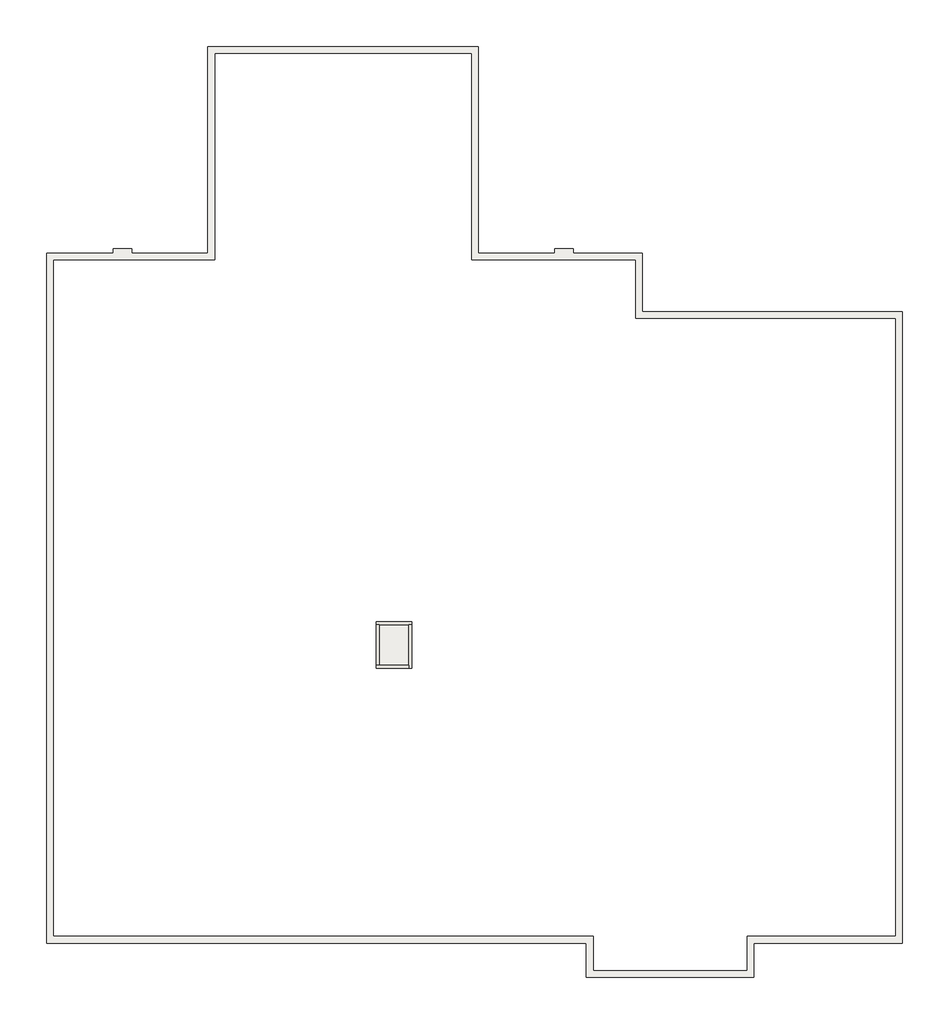
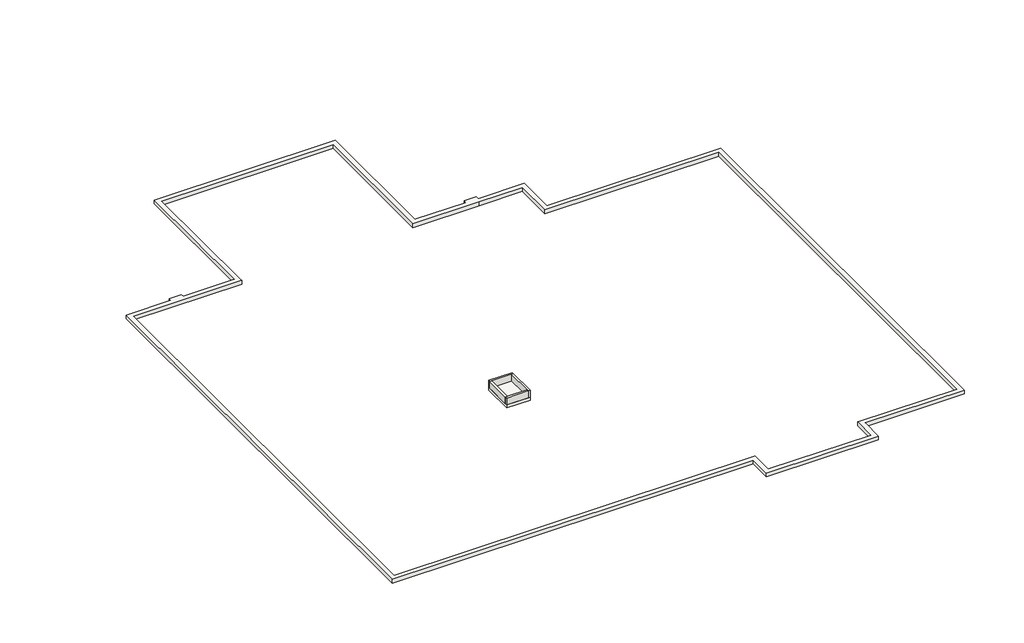
# One storey: 4 walls, 2 slabs.
"""IFC4 building model written with IfcOpenShell, lengths in millimetres."""

from ifc_helpers import new_model, si_unit, frame, origin, place, context, project, spatial, polyline, outline, extrude, faceted_brep, element, save

model = new_model("IFC4")

# Units and contexts
model_context = context("Model", 3, world=origin())
ifc_project = project(units=[si_unit("LENGTHUNIT", "METRE", prefix="MILLI")], contexts=[model_context])

# Site, building, storey
site = spatial("IfcSite", under=ifc_project)
building = spatial("IfcBuilding", under=site)
storey = spatial("IfcBuildingStorey", under=building, Name="02_FU_OKFU_-5,10__Aufzug", Elevation=-5100.0)

# Slabs
placement = place(None, origin())
element("IfcSlab", 1, ObjectType="5dki Aufzugsunterfahrt Bopla 40cm C40/50", at=placement, inside=storey, context=model_context, shape_type="SweptSolid", body=[
    extrude(outline(polyline([(30641.9991141, 10662.0130303), (30641.9991141, 6740.0014141), (27641.9992024, 6740.0014141), (27641.9992024, 10662.0130303), (30641.9991141, 10662.0130303)])), frame((0.0, 0.0, -5500.0), z_axis=(0.0, 0.0, 1.0), x_axis=(1.0, 0.0, 0.0)), (0.0, 0.0, 1.0), 400.0),
])
element("IfcSlab", 2, ObjectType="5dki Streifenfundament 50cm C100/115", at=placement, inside=storey, context=model_context, shape_type="SweptSolid", body=[
    extrude(outline(polyline([(13469.6232746, 59125.9283486), (36270.0003049, 59125.9283486), (36270.0003049, 41717.5032758), (42691.9991624, 41717.5032758), (42691.9991624, 42097.5032758), (44242.0014149, 42095.9282045), (44242.0014149, 41717.5032758), (50070.0000211, 41717.5032758), (50069.999894, 36785.573951), (71979.9986133, 36785.5734213), (71979.9986133, -16430.0005666), (59476.9100357, -16430.0005666), (59476.9100357, -19332.4966002), (45370.0202351, -19332.4966002), (45370.0202351, -16430.0005666), (-129.9986936, -16430.0005666), (-129.9986936, 41717.0011496), (5491.9984311, 41717.0011496), (5491.9984311, 42095.9291895), (7042.0004993, 42095.9291528), (7042.0004993, 41717.5032758), (13469.6232746, 41717.5032758), (13469.6232746, 59125.9283486)]), holes=[polyline([(35670.0003049, 58525.9283486), (14069.6232746, 58525.9283486), (14069.6232746, 41117.5032758), (470.0013064, 41117.5032758), (470.0013064, -15830.0005666), (45970.0202351, -15830.0005666), (45970.0202351, -18732.4966002), (58876.9100357, -18732.4966002), (58876.9100357, -15830.0005666), (71379.9986133, -15830.0005666), (71379.9986133, 36185.5734358), (49469.9998785, 36185.5739655), (49470.0000056, 41117.5032758), (44041.4717429, 41117.5032758), (35670.0003049, 41117.5032758), (35670.0003049, 58525.9283486)])]), frame((0.0, 0.0, -5100.0), z_axis=(0.0, 0.0, 1.0), x_axis=(1.0, 0.0, 0.0)), (0.0, 0.0, 1.0), 500.0),
])

# Walls
element("IfcWall", 3, ObjectType="5dki Aufzugsunterfahrt STB-Wand 25cm C40/50", at=placement, inside=storey, context=model_context, shape_type="Brep", body=[
    faceted_brep([(27641.9992024, 10412.0124709, -5100.0), (27891.9992024, 10412.0125176, -5100.0), (30385.8202349, 10412.0129836, -5100.0), (30635.8205887, 10412.0130303, -5100.0), (30635.8205887, 10412.0130303, -4200.0), (30385.8202349, 10412.0129836, -4200.0), (27891.9992024, 10412.0125176, -4200.0), (27641.9992024, 10412.0124709, -4200.0), (27641.9992024, 10662.0124709, -5100.0), (27641.9992024, 10662.0124709, -4200.0), (30635.3999388, 10662.0130303, -4200.0), (30635.3999388, 10662.0130303, -5100.0)], [[[0, 1, 2, 3, 4, 5, 6, 7]], [[8, 9, 10, 11]], [[3, 2, 1, 0, 8, 11]], [[7, 6, 5, 4, 10, 9]], [[4, 3, 11, 10]], [[0, 7, 9, 8]]]),
])
element("IfcWall", 4, ObjectType="5dki Aufzugsunterfahrt STB-Wand 25cm C40/50", at=placement, inside=storey, context=model_context, shape_type="Brep", body=[
    faceted_brep([(30385.8202349, 10412.0129836, -5100.0), (30391.5781103, 6990.0014141, -5100.0), (30391.9987602, 6740.0014141, -5100.0), (30391.9987602, 6740.0014141, -4200.0), (30391.5781103, 6990.0014141, -4200.0), (30385.8202349, 10412.0129836, -4200.0), (30635.8205887, 10412.0130303, -5100.0), (30635.8205887, 10412.0130303, -4200.0), (30641.9991141, 6740.0014141, -4200.0), (30641.9991141, 6740.0014141, -5100.0)], [[[0, 1, 2, 3, 4, 5]], [[6, 7, 8, 9]], [[2, 1, 0, 6, 9]], [[5, 4, 3, 8, 7]], [[0, 5, 7, 6]], [[3, 2, 9, 8]]]),
])
element("IfcWall", 5, ObjectType="5dki Aufzugsunterfahrt STB-Wand 25cm C40/50", at=placement, inside=storey, context=model_context, shape_type="Brep", body=[
    faceted_brep([(30391.5781103, 6990.0014141, -5100.0), (27891.9992024, 6990.0014141, -5100.0), (27641.9992024, 6990.0014141, -5100.0), (27641.9992024, 6990.0014141, -4200.0), (27891.9992024, 6990.0014141, -4200.0), (30391.5781103, 6990.0014141, -4200.0), (30391.9987602, 6740.0014141, -5100.0), (30391.9987602, 6740.0014141, -4200.0), (27641.9992024, 6740.0014141, -4200.0), (27641.9992024, 6740.0014141, -5100.0)], [[[0, 1, 2, 3, 4, 5]], [[6, 7, 8, 9]], [[2, 1, 0, 6, 9]], [[5, 4, 3, 8, 7]], [[0, 5, 7, 6]], [[3, 2, 9, 8]]]),
])
element("IfcWall", 6, ObjectType="5dki Aufzugsunterfahrt STB-Wand 25cm C40/50", at=placement, inside=storey, context=model_context, shape_type="SweptSolid", body=[
    extrude(outline(polyline([(27891.9992024, 10412.0125176), (27891.9992024, 6990.0014141), (27641.9992024, 6990.0014141), (27641.9992024, 10412.0124709), (27891.9992024, 10412.0125176)])), frame((0.0, 0.0, -5100.0), z_axis=(0.0, 0.0, 1.0), x_axis=(1.0, 0.0, 0.0)), (0.0, 0.0, 1.0), 900.0),
])

save(model, "model.ifc")

# Revit data of these elements
# Project information
#   StoreyModel = "<?xml version=\"1.0\" encoding=\"utf-16\"?>\n<StoreyModel xmlns:xsd=\"http://www.w3.org/2001/XMLSchema\" xmlns:xsi=\"http://www.w3.org/2001/XMLSchema-instance\" FormatVersion=\"2013.0.1.0\">\n  <GUID>d780c1b4-dd28-4844-915e-88a2c4b9528b</GUID>\n  <StoreyList />\n  <HelpLevelList />\n  <LastModificationDate>2014-08-27T10:30:40.9523468+02:00</LastModificationDate>\n  <LastModificationAutor>BiesingerMar</LastModificationAutor>\n  <SynchronizedStoreyModelFile />\n  <StandardConfiguration>\n    <Name>5D Standard</Name>\n    <Version>November 2012</Version>\n    <Description>5D-Standardkonfiguration</Description>\n    <LastModificationDate>2012-11-26T14:42:43.0850171+01:00</LastModificationDate>\n    <LastModificationAutor>5D-Administrator</LastModificationAutor>\n    <LevelStandard>\n      <LevelUsageList>\n        <LevelUsage>\n          <ID>0</ID>\n          <Function>Standard</Function>\n          <Name>STRD</Name>\n          <Abbreviation>STRD</Abbreviation>\n        </LevelUsage>\n        <LevelUsage>\n          <ID>1</ID>\n          <Function>Unterkante Rohdecke</Function>\n          <Name>UKRD</Name>\n          <Abbreviation>UKRD</Abbreviation>\n        </LevelUsage>\n        <LevelUsage>\n          <ID>2</ID>\n          <Function>Oberkante Rohdecke</Function>\n          <Name>OKRD</Name>\n          <Abbreviation>OKRD</Abbreviation>\n        </LevelUsage>\n        <LevelUsage>\n          <ID>3</ID>\n          <Function>Oberkante Fertigfußboden</Function>\n          <Name>OKFB</Name>\n          <Abbreviation>OKFB</Abbreviation>\n        </LevelUsage>\n        <LevelUsage>\n          <ID>4</ID>\n          <Function>Unterkante Abgehängter Decke</Function>\n          <Name>UKAD</Name>\n          <Abbreviation>UKAD</Abbreviation>\n        </LevelUsage>\n        <LevelUsage>\n          <ID>5</ID>\n          <Function>Statik</Function>\n          <Name>STAT</Name>\n          <Abbreviation>STAT</Abbreviation>\n        </LevelUsage>\n        <LevelUsage>\n          <ID>100</ID>\n          <Function>Hilfsebene</Function>\n          <Name>HELP</Name>\n          <Abbreviation>HELP</Abbreviation>\n        </LevelUsage>\n        <LevelUsage>\n          <ID>1000</ID>\n          <Function>Oberkante Fundament</Function>\n          <Name>OKFU</Name>\n          <Abbreviation>OKFU</Abbreviation>\n        </LevelUsage>\n        <LevelUsage>\n          <ID>1001</ID>\n          <Function>Unterkante Träger</Function>\n          <Name>UKTR</Name>\n          <Abbreviation>UKTR</Abbreviation>\n        </LevelUsage>\n        <LevelUsage>\n          <ID>1002</ID>\n          <Function>Lift</Function>\n          <Name>LIFT</Name>\n          <Abbreviation>LIFT</Abbreviation>\n        </LevelUsage>\n        <LevelUsage>\n          <ID>1003</ID>\n          <Function>Sockel</Function>\n          <Name>SOCK</Name>\n          <Abbreviation>SOCK</Abbreviation>\n        </LevelUsage>\n        <LevelUsage>\n          <ID>1004</ID>\n          <Function>Wandoberkante</Function>\n          <Name>OKWA</Name>\n          <Abbreviation>OKWA</Abbreviation>\n        </LevelUsage>\n        <LevelUsage>\n          <ID>1005</ID>\n          <Function>Dämmebene</Function>\n          <Name>DAEM</Name>\n          <Abbreviation>DAEM</Abbreviation>\n        </LevelUsage>\n        <LevelUsage>\n          <ID>1006</ID>\n          <Function>OK geneigtes Objekt</Function>\n          <Name>NEIG</Name>\n          <Abbreviation>NEIG</Abbreviation>\n        </LevelUsage>\n        <LevelUsage>\n          <ID>1007</ID>\n          <Function>Außenanlagen</Function>\n          <Name>AUSS</Name>\n          <Abbreviation>AUSS</Abbreviation>\n        </LevelUsage>\n        <LevelUsage>\n          <ID>1008</ID>\n          <Function>Boeschung Oberkante</Function>\n          <Name>BOOK</Name>\n          <Abbreviation>BOOK</Abbreviation>\n        </LevelUsage>\n        <LevelUsage>\n          <ID>1009</ID>\n          <Function>Boeschung Unterkante</Function>\n          <Name>BOUK</Name>\n          <Abbreviation>BOUK</Abbreviation>\n        </LevelUsage>\n        <LevelUsage>\n          <ID>1010</ID>\n          <Function>Treppe OK obere Ebene</Function>\n          <Name>TROK</Name>\n          <Abbreviation>TROK</Abbreviation>\n        </LevelUsage>\n        <LevelUsage>\n          <ID>1011</ID>\n          <Function>Treppe OK untere Ebene</Function>\n          <Name>TRUK</Name>\n          <Abbreviation>TRUK</Abbreviation>\n        </LevelUsage>\n        <LevelUsage>\n          <ID>1012</ID>\n          <Function>Treppe OK Podest 1</Function>\n          <Name>TRP1</Name>\n          <Abbreviation>TRP1</Abbreviation>\n        </LevelUsage>\n        <LevelUsage>\n          <ID>1013</ID>\n          <Function>Treppe OK Podest 2</Function>\n          <Name>TRP2</Name>\n          <Abbreviation>TRP2</Abbreviation>\n        </LevelUsage>\n        <LevelUsage>\n          <ID>1014</ID>\n          <Function>Unterkante Fundament</Function>\n          <Name>UKFU</Name>\n          <Abbreviation>UKFU</Abbreviation>\n        </LevelUsage>\n        <LevelUsage>\n          <ID>1015</ID>\n          <Function>Attika OK</Function>\n          <Name>ATOK</Name>\n          <Abbreviation>ATOK</Abbreviation>\n        </LevelUsage>\n        <LevelUsage>\n          <ID>1017</ID>\n          <Function>OK Vormauerung</Function>\n          <Name>OKVM</Name>\n          <Abbreviation>OKVM</Abbreviation>\n        </LevelUsage>\n        <LevelUsage>\n          <ID>1018</ID>\n          <Function>Lichtschacht Oberkante</Function>\n          <Name>LISO</Name>\n          <Abbreviation>LISO</Abbreviation>\n        </LevelUsage>\n        <LevelUsage>\n          <ID>1019</ID>\n          <Function>Unterkante Dämmung</Function>\n          <Name>DAEU</Name>\n          <Abbreviation>DAEU</Abbreviation>\n        </LevelUsage>\n      </LevelUsageList>\n      <DefaultLevelNameLogic>[Geschoss_FormatNummer]_[Geschoss_Verwendung_Kuerzel]_[Ebenen_Verwendung_Kuerzel]_[Ebenen_Projekthöhe]_[Ebenen_Kommentar]</DefaultLevelNameLogic>\n      <DefaultMainLevelUsage>3</DefaultMainLevelUsage>\n    </LevelStandard>\n    <StoreyStandard>\n      <DefaultStoreyNameLogic>[Geschoss_FormatNummer]_[Geschoss_Verwendung_Kuerzel]</DefaultStoreyNameLogic>\n      <StoreyUsageList>\n        <StoreyUsage>\n          <ID>0</ID>\n          <Function>Standard</Function>\n          <Name>Standard</Name>\n          <Abbreviation>ZZ</Abbreviation>\n        </StoreyUsage>\n        <StoreyUsage>\n          <ID>1</ID>\n          <Function>OberGeschoss</Function>\n          <Name>OberGeschoss</Name>\n          <Abbreviation>OG</Abbreviation>\n        </StoreyUsage>\n        <StoreyUsage>\n          <ID>2</ID>\n          <Function>UnterGeschoss</Function>\n          <Name>UnterGeschoss</Name>\n          <Abbreviation>UG</Abbreviation>\n        </StoreyUsage>\n        <StoreyUsage>\n          <ID>3</ID>\n          <Function>ErdGeschoss</Function>\n          <Name>ErdGeschoss</Name>\n          <Abbreviation>EG</Abbreviation>\n        </StoreyUsage>\n        <StoreyUsage>\n          <ID>4</ID>\n          <Function>DachGeschoss</Function>\n          <Name>DachGeschoss</Name>\n          <Abbreviation>DG</Abbreviation>\n        </StoreyUsage>\n        <StoreyUsage>\n          <ID>6</ID>\n          <Function>Keller</Function>\n          <Name>KellerGeschoss</Name>\n          <Abbreviation>KG</Abbreviation>\n        </StoreyUsage>\n        <StoreyUsage>\n          <ID>7</ID>\n          <Function>Tiefgarage</Function>\n          <Name>TiefgaragenGeschoss</Name>\n          <Abbreviation>TG</Abbreviation>\n        </StoreyUsage>\n        <StoreyUsage>\n          <ID>5</ID>\n          <Function>Technisches Geschoss</Function>\n          <Name>Technisches Geschoss</Name>\n          <Abbreviation>XG</Abbreviation>\n        </StoreyUsage>\n        <StoreyUsage>\n          <ID>1000</ID>\n          <Function>Treppenhaus</Function>\n          <Name>ZwischengGeschossTreppe</Name>\n          <Abbreviation>ZG</Abbreviation>\n        </StoreyUsage>\n        <StoreyUsage>\n          <ID>1001</ID>\n          <Function>Fundament</Function>\n          <Name>Fundament</Name>\n          <Abbreviation>FU</Abbreviation>\n        </StoreyUsage>\n        <StoreyUsage>\n          <ID>1002</ID>\n          <Function>Dachkonstruktion</Function>\n          <Name>Dachkonstruktion</Name>\n          <Abbreviation>DA</Abbreviation>\n        </StoreyUsage>\n        <StoreyUsage>\n          <ID>1004</ID>\n          <Function>Lift</Function>\n          <Name>Lift</Name>\n          <Abbreviation>LI</Abbreviation>\n        </StoreyUsage>\n      </StoreyUsageList>\n      <StoreyLocationList>\n        <StoreyLocation>\n          <ID>1</ID>\n          <Function>oberirdisch</Function>\n          <Name>oberirdisch</Name>\n          <Abbreviation />\n        </StoreyLocation>\n        <StoreyLocation>\n          <ID>2</ID>\n          <Function>unterirdisch</Function>\n          <Name>unterirdisch</Name>\n          <Abbreviation />\n        </StoreyLocation>\n      </StoreyLocationList>\n      <StoreyHeight>9.84251968503937</StoreyHeight>\n      <StoreyNumberOnOvergroundFormat>\n        <Digits>2</Digits>\n        <Prefix />\n        <Suffix />\n      </StoreyNumberOnOvergroundFormat>\n      <StoreyNumberOnUndergroundFormat>\n        <Digits>2</Digits>\n        <Prefix />\n        <Suffix />\n      </StoreyNumberOnUndergroundFormat>\n      <EntresolNumberFormat>\n        <Digits>2</Digits>\n        <Prefix />\n        <Suffix />\n      </EntresolNumberFormat>\n    </StoreyStandard>\n  </StandardConfiguration>\n  <RevisionNumber>35</RevisionNumber>\n  <WriteLock>false</WriteLock>\n</StoreyModel>"
#   BrowserStrukturXMLData = "<Browserstruktur>\n  <xs:schema id=\"Browserstruktur\" xmlns=\"\" xmlns:xs=\"http://www.w3.org/2001/XMLSchema\" xmlns:msdata=\"urn:schemas-microsoft-com:xml-msdata\">\n    <xs:element name=\"Browserstruktur\" msdata:IsDataSet=\"true\" msdata:MainDataTable=\"ViewTemplates\" msdata:UseCurrentLocale=\"true\">\n      <xs:complexType>\n        <xs:choice minOccurs=\"0\" maxOccurs=\"unbounded\">\n          <xs:element name=\"ViewTemplates\">\n            <xs:complexType>\n              <xs:sequence>\n                <xs:element name=\"Erstellen\" type=\"xs:boolean\" minOccurs=\"0\" />\n                <xs:element name=\"Ansichtsvorlage\" type=\"xs:string\" />\n                <xs:element name=\"_x0031__Fachbereich\" type=\"xs:string\" minOccurs=\"0\" />\n                <xs:element name=\"_x0032__Ansichtstyp\" type=\"xs:string\" minOccurs=\"0\" />\n                <xs:element name=\"_x0033__Ansichtsgruppe\" type=\"xs:string\" minOccurs=\"0\" />\n                <xs:element name=\"Typ\" type=\"xs:string\" minOccurs=\"0\" />\n                <xs:element name=\"Klasse\" type=\"xs:string\" minOccurs=\"0\" />\n                <xs:element name=\"Bedingung\" type=\"xs:string\" minOccurs=\"0\" />\n                <xs:element name=\"Ebenenbezug\" type=\"xs:int\" minOccurs=\"0\" />\n                <xs:element name=\"Ansichtsrichtung\" type=\"xs:string\" minOccurs=\"0\" />\n                <xs:element name=\"Ansichtsname\" type=\"xs:string\" minOccurs=\"0\" />\n              </xs:sequence>\n            </xs:complexType>\n          </xs:element>\n        </xs:choice>\n      </xs:complexType>\n      <xs:unique name=\"Constraint1\" msdata:PrimaryKey=\"true\">\n        <xs:selector xpath=\".//ViewTemplates\" />\n        <xs:field xpath=\"Ansichtsvorlage\" />\n      </xs:unique>\n    </xs:element>\n  </xs:schema>\n  <ViewTemplates>\n    <Erstellen>false</Erstellen>\n    <Ansichtsvorlage>010</Ansichtsvorlage>\n    <_x0031__Fachbereich>00_INTERN</_x0031__Fachbereich>\n    <_x0032__Ansichtstyp>010_CAD_UNTERLAGE</_x0032__Ansichtstyp>\n    <_x0033__Ansichtsgruppe>010_UNTERLAGE_CAD_GESAMT</_x0033__Ansichtsgruppe>\n    <Typ>FloorPlan</Typ>\n    <Klasse>ViewPlan</Klasse>\n    <Bedingung>einmalig</Bedingung>\n    <Ansichtsrichtung>&lt;Ignorieren&gt;</Ansichtsrichtung>\n    <Ansichtsname>[Geschoss_Name]_[Ansichtsgruppe_Name]_[Ebenen_Kommentar]</Ansichtsname>\n  </ViewTemplates>\n  <ViewTemplates>\n    <Erstellen>false</Erstellen>\n    <Ansichtsvorlage>011</Ansichtsvorlage>\n    <_x0031__Fachbereich>00_INTERN</_x0031__Fachbereich>\n    <_x0032__Ansichtstyp>010_CAD_UNTERLAGE</_x0032__Ansichtstyp>\n    <_x0033__Ansichtsgruppe>011_LAGEPLAN</_x0033__Ansichtsgruppe>\n    <Typ>FloorPlan</Typ>\n    <Klasse>ViewPlan</Klasse>\n    <Bedingung>einmalig</Bedingung>\n    <Ansichtsrichtung>&lt;Ignorieren&gt;</Ansichtsrichtung>\n    <Ansichtsname>[Geschoss_Name]_[Ansichtsgruppe_Name]_[Ebenen_Kommentar]</Ansichtsname>\n  </ViewTemplates>\n  <ViewTemplates>\n    <Erstellen>false</Erstellen>\n    <Ansichtsvorlage>025</Ansichtsvorlage>\n    <_x0031__Fachbereich>00_INTERN</_x0031__Fachbereich>\n    <_x0032__Ansichtstyp>010_CAD_UNTERLAGE</_x0032__Ansichtstyp>\n    <_x0033__Ansichtsgruppe>025_ACHSEN</_x0033__Ansichtsgruppe>\n    <Typ>FloorPlan</Typ>\n    <Klasse>ViewPlan</Klasse>\n    <Bedingung>einmalig</Bedingung>\n    <Ansichtsrichtung>&lt;Ignorieren&gt;</Ansichtsrichtung>\n    <Ansichtsname>[Geschoss_Name]_[Ansichtsgruppe_Name]_[Ebenen_Kommentar]</Ansichtsname>\n  </ViewTemplates>\n  <ViewTemplates>\n    <Erstellen>false</Erstellen>\n    <Ansichtsvorlage>030</Ansichtsvorlage>\n    <_x0031__Fachbereich>00_INTERN</_x0031__Fachbereich>\n    <_x0032__Ansichtstyp>010_CAD_UNTERLAGE</_x0032__Ansichtstyp>\n    <_x0033__Ansichtsgruppe>030_ENTWURF_ARCHITEKT</_x0033__Ansichtsgruppe>\n    <Typ>FloorPlan</Typ>\n    <Klasse>ViewPlan</Klasse>\n    <Bedingung>einmalig</Bedingung>\n    <Ebenenbezug>100</Ebenenbezug>\n    <Ansichtsrichtung>&lt;Ignorieren&gt;</Ansichtsrichtung>\n    <Ansichtsname>[Geschoss_Name]_[Ansichtsgruppe_Name]_[Ebenen_Kommentar]</Ansichtsname>\n  </ViewTemplates>\n  <ViewTemplates>\n    <Erstellen>false</Erstellen>\n    <Ansichtsvorlage>060</Ansichtsvorlage>\n    <_x0031__Fachbereich>00_INTERN</_x0031__Fachbereich>\n    <_x0032__Ansichtstyp>060_BILD_UNTERLAGE</_x0032__Ansichtstyp>\n    <_x0033__Ansichtsgruppe>060_UNTERLAGE_BITMAP</_x0033__Ansichtsgruppe>\n    <Typ>FloorPlan</Typ>\n    <Klasse>ViewPlan</Klasse>\n    <Bedingung>einmalig</Bedingung>\n    <Ansichtsrichtung>&lt;Ignorieren&gt;</Ansichtsrichtung>\n    <Ansichtsname>[Geschoss_Name]_[Ansichtsgruppe_Name]_[Ebenen_Kommentar]</Ansichtsname>\n  </ViewTemplates>\n  <ViewTemplates>\n    <Erstellen>false</Erstellen>\n    <Ansichtsvorlage>070</Ansichtsvorlage>\n    <_x0031__Fachbereich>00_INTERN</_x0031__Fachbereich>\n    <_x0032__Ansichtstyp>070_CAD_UEBERLAGE</_x0032__Ansichtstyp>\n    <_x0033__Ansichtsgruppe>070_UEBERLAGE_CAD</_x0033__Ansichtsgruppe>\n    <Typ>FloorPlan</Typ>\n    <Klasse>ViewPlan</Klasse>\n    <Bedingung>einmalig</Bedingung>\n    <Ansichtsrichtung>&lt;Ignorieren&gt;</Ansichtsrichtung>\n    <Ansichtsname>[Geschoss_Name]_[Ansichtsgruppe_Name]_[Ebenen_Kommentar]</Ansichtsname>\n  </ViewTemplates>\n  <ViewTemplates>\n    <Erstellen>false</Erstellen>\n    <Ansichtsvorlage>080</Ansichtsvorlage>\n    <_x0031__Fachbereich>00_INTERN</_x0031__Fachbereich>\n    <_x0032__Ansichtstyp>080_BILD_UEBERLAGE</_x0032__Ansichtstyp>\n    <_x0033__Ansichtsgruppe>080_UEBERLAGE_BITMAP</_x0033__Ansichtsgruppe>\n    <Typ>FloorPlan</Typ>\n    <Klasse>ViewPlan</Klasse>\n    <Bedingung>einmalig</Bedingung>\n    <Ansichtsrichtung>&lt;Ignorieren&gt;</Ansichtsrichtung>\n    <Ansichtsname>[Geschoss_Name]_[Ansichtsgruppe_Name]_[Ebenen_Kommentar]</Ansichtsname>\n  </ViewTemplates>\n  <ViewTemplates>\n    <Erstellen>false</Erstellen>\n    <Ansichtsvorlage>K_5_CC</Ansichtsvorlage>\n    <_x0031__Fachbereich>K_KONSTRUKTION</_x0031__Fachbereich>\n    <_x0032__Ansichtstyp>5_INGENIEUR / ROHBAU</_x0032__Ansichtstyp>\n    <_x0033__Ansichtsgruppe>5_CC_WÄNDE/STÜTZEN</_x0033__Ansichtsgruppe>\n    <Typ>FloorPlan</Typ>\n    <Klasse>ViewPlan</Klasse>\n    <Bedingung>Für jedes Geschoß</Bedingung>\n    <Ebenenbezug>-2</Ebenenbezug>\n    <Ansichtsrichtung>&lt;Ignorieren&gt;</Ansichtsrichtung>\n    <Ansichtsname>[Geschoss_Name]_[Ansichtsgruppe_Name]_[Ebenen_Kommentar]</Ansichtsname>\n  </ViewTemplates>\n  <ViewTemplates>\n    <Erstellen>false</Erstellen>\n    <Ansichtsvorlage>K_5_AA</Ansichtsvorlage>\n    <_x0031__Fachbereich>K_KONSTRUKTION</_x0031__Fachbereich>\n    <_x0032__Ansichtstyp>5_INGENIEUR / ROHBAU</_x0032__Ansichtstyp>\n    <_x0033__Ansichtsgruppe>5_AA_FUNDAMENTE</_x0033__Ansichtsgruppe>\n    <Typ>FloorPlan</Typ>\n    <Klasse>ViewPlan</Klasse>\n    <Bedingung>Für jedes Geschoß</Bedingung>\n    <Ebenenbezug>1000</Ebenenbezug>\n    <Ansichtsrichtung>&lt;Ignorieren&gt;</Ansichtsrichtung>\n    <Ansichtsname>[Geschoss_Name]_[Ansichtsgruppe_Name]_[Ebenen_Kommentar]</Ansichtsname>\n  </ViewTemplates>\n  <ViewTemplates>\n    <Erstellen>false</Erstellen>\n    <Ansichtsvorlage>K_5_BB</Ansichtsvorlage>\n    <_x0031__Fachbereich>K_KONSTRUKTION</_x0031__Fachbereich>\n    <_x0032__Ansichtstyp>5_INGENIEUR / ROHBAU</_x0032__Ansichtstyp>\n    <_x0033__Ansichtsgruppe>5_BB_BODENPLATTE</_x0033__Ansichtsgruppe>\n    <Typ>FloorPlan</Typ>\n    <Klasse>ViewPlan</Klasse>\n    <Bedingung>Für jedes Geschoß</Bedingung>\n    <Ebenenbezug>2</Ebenenbezug>\n    <Ansichtsrichtung>&lt;Ignorieren&gt;</Ansichtsrichtung>\n    <Ansichtsname>[Geschoss_Name]_[Ansichtsgruppe_Name]_[Ebenen_Kommentar]</Ansichtsname>\n  </ViewTemplates>\n  <ViewTemplates>\n    <Erstellen>false</Erstellen>\n    <Ansichtsvorlage>K_5_EE</Ansichtsvorlage>\n    <_x0031__Fachbereich>K_KONSTRUKTION</_x0031__Fachbereich>\n    <_x0032__Ansichtstyp>5_INGENIEUR / ROHBAU</_x0032__Ansichtstyp>\n    <_x0033__Ansichtsgruppe>5_EE_GESCHOSSDECKEN</_x0033__Ansichtsgruppe>\n    <Typ>FloorPlan</Typ>\n    <Klasse>ViewPlan</Klasse>\n    <Bedingung>Für jedes Geschoß</Bedingung>\n    <Ebenenbezug>2</Ebenenbezug>\n    <Ansichtsrichtung>&lt;Ignorieren&gt;</Ansichtsrichtung>\n    <Ansichtsname>[Geschoss_Name]_[Ansichtsgruppe_Name]_[Ebenen_Kommentar]</Ansichtsname>\n  </ViewTemplates>\n  <ViewTemplates>\n    <Erstellen>false</Erstellen>\n    <Ansichtsvorlage>K_6b_AA</Ansichtsvorlage>\n    <_x0031__Fachbereich>K_KONSTRUKTION</_x0031__Fachbereich>\n    <_x0032__Ansichtstyp>6b_FASSADE</_x0032__Ansichtstyp>\n    <_x0033__Ansichtsgruppe>6b_AA_FENSTER_UND_GLASFASSADE</_x0033__Ansichtsgruppe>\n    <Typ>FloorPlan</Typ>\n    <Klasse>ViewPlan</Klasse>\n    <Bedingung>Für jedes Geschoß</Bedingung>\n    <Ebenenbezug>-2</Ebenenbezug>\n    <Ansichtsrichtung>&lt;Ignorieren&gt;</Ansichtsrichtung>\n    <Ansichtsname>[Geschoss_Name]_[Ansichtsgruppe_Name]_[Ebenen_Kommentar]</Ansichtsname>\n  </ViewTemplates>\n  <ViewTemplates>\n    <Erstellen>false</Erstellen>\n    <Ansichtsvorlage>K_6b_DD</Ansichtsvorlage>\n    <_x0031__Fachbereich>K_KONSTRUKTION</_x0031__Fachbereich>\n    <_x0032__Ansichtstyp>6b_FASSADE</_x0032__Ansichtstyp>\n    <_x0033__Ansichtsgruppe>6b_DD_AUßENPUTZ_WDVS</_x0033__Ansichtsgruppe>\n    <Typ>FloorPlan</Typ>\n    <Klasse>ViewPlan</Klasse>\n    <Bedingung>Für jedes Geschoß</Bedingung>\n    <Ebenenbezug>-2</Ebenenbezug>\n    <Ansichtsrichtung>&lt;Ignorieren&gt;</Ansichtsrichtung>\n    <Ansichtsname>[Geschoss_Name]_[Ansichtsgruppe_Name]_[Ebenen_Kommentar]</Ansichtsname>\n  </ViewTemplates>\n  <ViewTemplates>\n    <Erstellen>false</Erstellen>\n    <Ansichtsvorlage>K_5_S1_AA</Ansichtsvorlage>\n    <_x0031__Fachbereich>K_KONSTRUKTION</_x0031__Fachbereich>\n    <_x0032__Ansichtstyp>5_S1_STATIK</_x0032__Ansichtstyp>\n    <_x0033__Ansichtsgruppe>5_S1_AA_GRUNDRISSE</_x0033__Ansichtsgruppe>\n    <Typ>FloorPlan</Typ>\n    <Klasse>ViewPlan</Klasse>\n    <Bedingung>Für jedes Geschoß</Bedingung>\n    <Ebenenbezug>-2</Ebenenbezug>\n    <Ansichtsrichtung>&lt;Ignorieren&gt;</Ansichtsrichtung>\n    <Ansichtsname>[Geschoss_Name]_[Ansichtsgruppe_Name]_[Ebenen_Kommentar]</Ansichtsname>\n  </ViewTemplates>\n  <ViewTemplates>\n    <Erstellen>false</Erstellen>\n    <Ansichtsvorlage>K_5_S2_AA</Ansichtsvorlage>\n    <_x0031__Fachbereich>K_KONSTRUKTION</_x0031__Fachbereich>\n    <_x0032__Ansichtstyp>5_S2_BEWEHRUNG</_x0032__Ansichtstyp>\n    <_x0033__Ansichtsgruppe>5_S2_AA_GRUNDRISSE</_x0033__Ansichtsgruppe>\n    <Typ>FloorPlan</Typ>\n    <Klasse>ViewPlan</Klasse>\n    <Bedingung>Für jedes Geschoß</Bedingung>\n    <Ebenenbezug>-2</Ebenenbezug>\n    <Ansichtsrichtung>&lt;Ignorieren&gt;</Ansichtsrichtung>\n    <Ansichtsname>[Geschoss_Name]_[Ansichtsgruppe_Name]_[Ebenen_Kommentar]</Ansichtsname>\n  </ViewTemplates>\n  <ViewTemplates>\n    <Erstellen>false</Erstellen>\n    <Ansichtsvorlage>K_5_DD</Ansichtsvorlage>\n    <_x0031__Fachbereich>K_KONSTRUKTION</_x0031__Fachbereich>\n    <_x0032__Ansichtstyp>5_INGENIEUR / ROHBAU</_x0032__Ansichtstyp>\n    <_x0033__Ansichtsgruppe>5_DD_TRÄGER</_x0033__Ansichtsgruppe>\n    <Typ>FloorPlan</Typ>\n    <Klasse>ViewPlan</Klasse>\n    <Bedingung>Für jedes Geschoß</Bedingung>\n    <Ebenenbezug>1</Ebenenbezug>\n    <Ansichtsrichtung>&lt;Ignorieren&gt;</Ansichtsrichtung>\n    <Ansichtsname>[Geschoss_Name]_[Ansichtsgruppe_Name]_[Ebenen_Kommentar]</Ansichtsname>\n  </ViewTemplates>\n  <ViewTemplates>\n    <Erstellen>false</Erstellen>\n    <Ansichtsvorlage>K_5_S1_BB</Ansichtsvorlage>\n    <_x0031__Fachbereich>K_KONSTRUKTION</_x0031__Fachbereich>\n    <_x0032__Ansichtstyp>5_S1_STATIK</_x0032__Ansichtstyp>\n    <_x0033__Ansichtsgruppe>5_S1_BB_DECKENSPIEGEL</_x0033__Ansichtsgruppe>\n    <Typ>FloorPlan</Typ>\n    <Klasse>ViewPlan</Klasse>\n    <Bedingung>Für jedes Geschoß</Bedingung>\n    <Ebenenbezug>2</Ebenenbezug>\n    <Ansichtsrichtung>&lt;Ignorieren&gt;</Ansichtsrichtung>\n    <Ansichtsname>[Geschoss_Name]_[Ansichtsgruppe_Name]_[Ebenen_Kommentar]</Ansichtsname>\n  </ViewTemplates>\n  <ViewTemplates>\n    <Erstellen>false</Erstellen>\n    <Ansichtsvor
#     lage>K_5_S2_BB</Ansichtsvorlage>\n    <_x0031__Fachbereich>K_KONSTRUKTION</_x0031__Fachbereich>\n    <_x0032__Ansichtstyp>5_S2_BEWEHRUNG</_x0032__Ansichtstyp>\n    <_x0033__Ansichtsgruppe>5_S2_BB_DECKENSPIEGEL</_x0033__Ansichtsgruppe>\n    <Typ>FloorPlan</Typ>\n    <Klasse>ViewPlan</Klasse>\n    <Bedingung>Für jedes Geschoß</Bedingung>\n    <Ebenenbezug>2</Ebenenbezug>\n    <Ansichtsrichtung>&lt;Ignorieren&gt;</Ansichtsrichtung>\n    <Ansichtsname>[Geschoss_Name]_[Ansichtsgruppe_Name]_[Ebenen_Kommentar]</Ansichtsname>\n  </ViewTemplates>\n  <ViewTemplates>\n    <Erstellen>false</Erstellen>\n    <Ansichtsvorlage>K_6b_BB</Ansichtsvorlage>\n    <_x0031__Fachbereich>K_KONSTRUKTION</_x0031__Fachbereich>\n    <_x0032__Ansichtstyp>6b_FASSADE</_x0032__Ansichtstyp>\n    <_x0033__Ansichtsgruppe>6b_BB_FASSADENBEKLEIDUNG</_x0033__Ansichtsgruppe>\n    <Typ>FloorPlan</Typ>\n    <Klasse>ViewPlan</Klasse>\n    <Bedingung>Für jedes Geschoß</Bedingung>\n    <Ebenenbezug>2</Ebenenbezug>\n    <Ansichtsrichtung>&lt;Ignorieren&gt;</Ansichtsrichtung>\n    <Ansichtsname>[Geschoss_Name]_[Ansichtsgruppe_Name]_[Ebenen_Kommentar]</Ansichtsname>\n  </ViewTemplates>\n  <ViewTemplates>\n    <Erstellen>false</Erstellen>\n    <Ansichtsvorlage>K_6b_CC</Ansichtsvorlage>\n    <_x0031__Fachbereich>K_KONSTRUKTION</_x0031__Fachbereich>\n    <_x0032__Ansichtstyp>6b_FASSADE</_x0032__Ansichtstyp>\n    <_x0033__Ansichtsgruppe>6b_CC_SONNENSCHUTZ_BLENDSCHUTZ</_x0033__Ansichtsgruppe>\n    <Typ>FloorPlan</Typ>\n    <Klasse>ViewPlan</Klasse>\n    <Bedingung>Für jedes Geschoß</Bedingung>\n    <Ebenenbezug>2</Ebenenbezug>\n    <Ansichtsrichtung>&lt;Ignorieren&gt;</Ansichtsrichtung>\n    <Ansichtsname>[Geschoss_Name]_[Ansichtsgruppe_Name]_[Ebenen_Kommentar]</Ansichtsname>\n  </ViewTemplates>\n  <ViewTemplates>\n    <Erstellen>false</Erstellen>\n    <Ansichtsvorlage>K_6c_AA</Ansichtsvorlage>\n    <_x0031__Fachbereich>K_KONSTRUKTION</_x0031__Fachbereich>\n    <_x0032__Ansichtstyp>6c_AUSBAU</_x0032__Ansichtstyp>\n    <_x0033__Ansichtsgruppe>6c_AA_WÄNDE_ALLGEMEIN</_x0033__Ansichtsgruppe>\n    <Typ>FloorPlan</Typ>\n    <Klasse>ViewPlan</Klasse>\n    <Bedingung>Für jedes Geschoß</Bedingung>\n    <Ebenenbezug>-2</Ebenenbezug>\n    <Ansichtsrichtung>&lt;Ignorieren&gt;</Ansichtsrichtung>\n    <Ansichtsname>[Geschoss_Name]_[Ansichtsgruppe_Name]_[Ebenen_Kommentar]</Ansichtsname>\n  </ViewTemplates>\n  <ViewTemplates>\n    <Erstellen>false</Erstellen>\n    <Ansichtsvorlage>K_6c_AC</Ansichtsvorlage>\n    <_x0031__Fachbereich>K_KONSTRUKTION</_x0031__Fachbereich>\n    <_x0032__Ansichtstyp>6c_AUSBAU</_x0032__Ansichtstyp>\n    <_x0033__Ansichtsgruppe>6c_AC_SYSTEMTRENNWÄNDE</_x0033__Ansichtsgruppe>\n    <Typ>FloorPlan</Typ>\n    <Klasse>ViewPlan</Klasse>\n    <Bedingung>Für jedes Geschoß</Bedingung>\n    <Ebenenbezug>3</Ebenenbezug>\n    <Ansichtsrichtung>&lt;Ignorieren&gt;</Ansichtsrichtung>\n    <Ansichtsname>[Geschoss_Name]_[Ansichtsgruppe_Name]_[Ebenen_Kommentar]</Ansichtsname>\n  </ViewTemplates>\n  <ViewTemplates>\n    <Erstellen>false</Erstellen>\n    <Ansichtsvorlage>K_6c_BX</Ansichtsvorlage>\n    <_x0031__Fachbereich>K_KONSTRUKTION</_x0031__Fachbereich>\n    <_x0032__Ansichtstyp>6c_AUSBAU</_x0032__Ansichtstyp>\n    <_x0033__Ansichtsgruppe>6c_BX_RÄUME (RAUMBEZEICHNUNGEN)</_x0033__Ansichtsgruppe>\n    <Typ>FloorPlan</Typ>\n    <Klasse>ViewPlan</Klasse>\n    <Bedingung>Für jedes Geschoß</Bedingung>\n    <Ebenenbezug>3</Ebenenbezug>\n    <Ansichtsrichtung>&lt;Ignorieren&gt;</Ansichtsrichtung>\n    <Ansichtsname>[Geschoss_Name]_[Ansichtsgruppe_Name]_[Ebenen_Kommentar]</Ansichtsname>\n  </ViewTemplates>\n  <ViewTemplates>\n    <Erstellen>false</Erstellen>\n    <Ansichtsvorlage>K_6c_BY</Ansichtsvorlage>\n    <_x0031__Fachbereich>K_KONSTRUKTION</_x0031__Fachbereich>\n    <_x0032__Ansichtstyp>6c_AUSBAU</_x0032__Ansichtstyp>\n    <_x0033__Ansichtsgruppe>6c_BY_RÄUME (NUTZFLÄCHEN NACH DIN 277)</_x0033__Ansichtsgruppe>\n    <Typ>FloorPlan</Typ>\n    <Klasse>ViewPlan</Klasse>\n    <Bedingung>Für jedes Geschoß</Bedingung>\n    <Ebenenbezug>3</Ebenenbezug>\n    <Ansichtsrichtung>&lt;Ignorieren&gt;</Ansichtsrichtung>\n    <Ansichtsname>[Geschoss_Name]_[Ansichtsgruppe_Name]_[Ebenen_Kommentar]</Ansichtsname>\n  </ViewTemplates>\n  <ViewTemplates>\n    <Erstellen>false</Erstellen>\n    <Ansichtsvorlage>K_6c_CA</Ansichtsvorlage>\n    <_x0031__Fachbereich>K_KONSTRUKTION</_x0031__Fachbereich>\n    <_x0032__Ansichtstyp>6c_AUSBAU</_x0032__Ansichtstyp>\n    <_x0033__Ansichtsgruppe>6c_CA_TÜREN_ALLGEMEIN</_x0033__Ansichtsgruppe>\n    <Typ>FloorPlan</Typ>\n    <Klasse>ViewPlan</Klasse>\n    <Bedingung>Für jedes Geschoß</Bedingung>\n    <Ebenenbezug>-2</Ebenenbezug>\n    <Ansichtsrichtung>&lt;Ignorieren&gt;</Ansichtsrichtung>\n    <Ansichtsname>[Geschoss_Name]_[Ansichtsgruppe_Name]_[Ebenen_Kommentar]</Ansichtsname>\n  </ViewTemplates>\n  <ViewTemplates>\n    <Erstellen>false</Erstellen>\n    <Ansichtsvorlage>K_6c_CB</Ansichtsvorlage>\n    <_x0031__Fachbereich>K_KONSTRUKTION</_x0031__Fachbereich>\n    <_x0032__Ansichtstyp>6c_AUSBAU</_x0032__Ansichtstyp>\n    <_x0033__Ansichtsgruppe>6c_CB_HOLZTÜREN (TYPEN)</_x0033__Ansichtsgruppe>\n    <Typ>FloorPlan</Typ>\n    <Klasse>ViewPlan</Klasse>\n    <Bedingung>Für jedes Geschoß</Bedingung>\n    <Ebenenbezug>-2</Ebenenbezug>\n    <Ansichtsrichtung>&lt;Ignorieren&gt;</Ansichtsrichtung>\n    <Ansichtsname>[Geschoss_Name]_[Ansichtsgruppe_Name]_[Ebenen_Kommentar]</Ansichtsname>\n  </ViewTemplates>\n  <ViewTemplates>\n    <Erstellen>false</Erstellen>\n    <Ansichtsvorlage>K_6c_CC</Ansichtsvorlage>\n    <_x0031__Fachbereich>K_KONSTRUKTION</_x0031__Fachbereich>\n    <_x0032__Ansichtstyp>6c_AUSBAU</_x0032__Ansichtstyp>\n    <_x0033__Ansichtsgruppe>6c_CC_BLECHTÜREN (TYPEN)</_x0033__Ansichtsgruppe>\n    <Typ>FloorPlan</Typ>\n    <Klasse>ViewPlan</Klasse>\n    <Bedingung>Für jedes Geschoß</Bedingung>\n    <Ebenenbezug>-2</Ebenenbezug>\n    <Ansichtsrichtung>&lt;Ignorieren&gt;</Ansichtsrichtung>\n    <Ansichtsname>[Geschoss_Name]_[Ansichtsgruppe_Name]_[Ebenen_Kommentar]</Ansichtsname>\n  </ViewTemplates>\n  <ViewTemplates>\n    <Erstellen>false</Erstellen>\n    <Ansichtsvorlage>K_6c_CD</Ansichtsvorlage>\n    <_x0031__Fachbereich>K_KONSTRUKTION</_x0031__Fachbereich>\n    <_x0032__Ansichtstyp>6c_AUSBAU</_x0032__Ansichtstyp>\n    <_x0033__Ansichtsgruppe>6c_CD_ROHRRAHMENTÜREN (TYPEN)</_x0033__Ansichtsgruppe>\n    <Typ>FloorPlan</Typ>\n    <Klasse>ViewPlan</Klasse>\n    <Bedingung>Für jedes Geschoß</Bedingung>\n    <Ebenenbezug>-2</Ebenenbezug>\n    <Ansichtsrichtung>&lt;Ignorieren&gt;</Ansichtsrichtung>\n    <Ansichtsname>[Geschoss_Name]_[Ansichtsgruppe_Name]_[Ebenen_Kommentar]</Ansichtsname>\n  </ViewTemplates>\n  <ViewTemplates>\n    <Erstellen>false</Erstellen>\n    <Ansichtsvorlage>K_6c_CE</Ansichtsvorlage>\n    <_x0031__Fachbereich>K_KONSTRUKTION</_x0031__Fachbereich>\n    <_x0032__Ansichtstyp>6c_AUSBAU</_x0032__Ansichtstyp>\n    <_x0033__Ansichtsgruppe>6c_CE_SPEZIALTÜREN/TORE</_x0033__Ansichtsgruppe>\n    <Typ>FloorPlan</Typ>\n    <Klasse>ViewPlan</Klasse>\n    <Bedingung>Für jedes Geschoß</Bedingung>\n    <Ebenenbezug>-2</Ebenenbezug>\n    <Ansichtsrichtung>&lt;Ignorieren&gt;</Ansichtsrichtung>\n    <Ansichtsname>[Geschoss_Name]_[Ansichtsgruppe_Name]_[Ebenen_Kommentar]</Ansichtsname>\n  </ViewTemplates>\n  <ViewTemplates>\n    <Erstellen>false</Erstellen>\n    <Ansichtsvorlage>K_6c_DA</Ansichtsvorlage>\n    <_x0031__Fachbereich>K_KONSTRUKTION</_x0031__Fachbereich>\n    <_x0032__Ansichtstyp>6c_AUSBAU</_x0032__Ansichtstyp>\n    <_x0033__Ansichtsgruppe>6c_DA_BODENKONSTRUKTION (TYPEN)</_x0033__Ansichtsgruppe>\n    <Typ>FloorPlan</Typ>\n    <Klasse>ViewPlan</Klasse>\n    <Bedingung>Für jedes Geschoß</Bedingung>\n    <Ebenenbezug>3</Ebenenbezug>\n    <Ansichtsrichtung>&lt;Ignorieren&gt;</Ansichtsrichtung>\n    <Ansichtsname>[Geschoss_Name]_[Ansichtsgruppe_Name]_[Ebenen_Kommentar]</Ansichtsname>\n  </ViewTemplates>\n  <ViewTemplates>\n    <Erstellen>false</Erstellen>\n    <Ansichtsvorlage>K_6c_AD</Ansichtsvorlage>\n    <_x0031__Fachbereich>K_KONSTRUKTION</_x0031__Fachbereich>\n    <_x0032__Ansichtstyp>6c_AUSBAU</_x0032__Ansichtstyp>\n    <_x0033__Ansichtsgruppe>6c_AD_WC_TRENNWÄNDE</_x0033__Ansichtsgruppe>\n    <Typ>FloorPlan</Typ>\n    <Klasse>ViewPlan</Klasse>\n    <Bedingung>Für jedes Geschoß</Bedingung>\n    <Ebenenbezug>3</Ebenenbezug>\n    <Ansichtsrichtung>&lt;Ignorieren&gt;</Ansichtsrichtung>\n    <Ansichtsname>[Geschoss_Name]_[Ansichtsgruppe_Name]_[Ebenen_Kommentar]</Ansichtsname>\n  </ViewTemplates>\n  <ViewTemplates>\n    <Erstellen>false</Erstellen>\n    <Ansichtsvorlage>K_5_FF</Ansichtsvorlage>\n    <_x0031__Fachbereich>K_KONSTRUKTION</_x0031__Fachbereich>\n    <_x0032__Ansichtstyp>5_INGENIEUR / ROHBAU</_x0032__Ansichtstyp>\n    <_x0033__Ansichtsgruppe>5_FF_EINBAUTEILE</_x0033__Ansichtsgruppe>\n    <Typ>FloorPlan</Typ>\n    <Klasse>ViewPlan</Klasse>\n    <Bedingung>Auswahl</Bedingung>\n    <Ebenenbezug>2</Ebenenbezug>\n    <Ansichtsrichtung>&lt;Ignorieren&gt;</Ansichtsrichtung>\n    <Ansichtsname>[Geschoss_Name]_[Ansichtsgruppe_Name]_[Ebenen_Kommentar]</Ansichtsname>\n  </ViewTemplates>\n  <ViewTemplates>\n    <Erstellen>false</Erstellen>\n    <Ansichtsvorlage>K_5_GG</Ansichtsvorlage>\n    <_x0031__Fachbereich>K_KONSTRUKTION</_x0031__Fachbereich>\n    <_x0032__Ansichtstyp>5_INGENIEUR / ROHBAU</_x0032__Ansichtstyp>\n    <_x0033__Ansichtsgruppe>5_GG_SONSTIGE_BAUTEILE</_x0033__Ansichtsgruppe>\n    <Typ>FloorPlan</Typ>\n    <Klasse>ViewPlan</Klasse>\n    <Bedingung>Auswahl</Bedingung>\n    <Ebenenbezug>2</Ebenenbezug>\n    <Ansichtsrichtung>&lt;Ignorieren&gt;</Ansichtsrichtung>\n    <Ansichtsname>[Geschoss_Name]_[Ansichtsgruppe_Name]_[Ebenen_Kommentar]</Ansichtsname>\n  </ViewTemplates>\n  <ViewTemplates>\n    <Erstellen>false</Erstellen>\n    <Ansichtsvorlage>K_6c_AE</Ansichtsvorlage>\n    <_x0031__Fachbereich>K_KONSTRUKTION</_x0031__Fachbereich>\n    <_x0032__Ansichtstyp>6c_AUSBAU</_x0032__Ansichtstyp>\n    <_x0033__Ansichtsgruppe>6c_AE_KELLER</_x0033__Ansichtsgruppe>\n    <Typ>FloorPlan</Typ>\n    <Klasse>ViewPlan</Klasse>\n    <Bedingung>Für jedes Geschoß</Bedingung>\n    <Ebenenbezug>3</Ebenenbezug>\n    <Ansichtsrichtung>&lt;Ignorieren&gt;</Ansichtsrichtung>\n    <Ansichtsname>[Geschoss_Name]_[Ansichtsgruppe_Name]_[Ebenen_Kommentar]</Ansichtsname>\n  </ViewTemplates>\n  <ViewTemplates>\n    <Erstellen>false</Erstellen>\n    <Ansichtsvorlage>K_6c_BA</Ansichtsvorlage>\n    <_x0031__Fachbereich>K_KONSTRUKTION</_x0031__Fachbereich>\n    <_x0032__Ansichtstyp>6c_AUSBAU</_x0032__Ansichtstyp>\n    <_x0033__Ansichtsgruppe>6c_BA_RÄUME (TYPEN)</_x0033__Ansichtsgruppe>\n    <Typ>FloorPlan</Typ>\n    <Klasse>ViewPlan</Klasse>\n    <Bedingung>Für jedes Geschoß</Bedingung>\n    <Ebenenbezug>3</Ebenenbezug>\n    <Ansichtsrichtung>&lt;Ignorieren&gt;</Ansichtsrichtung>\n    <Ansichtsname>[Geschoss_Name]_[Ansichtsgruppe_Name]_[Ebenen_Kommentar]</Ansichtsname>\n  </ViewTemplates>\n  <ViewTemplates>\n    <Erstellen>false</Erstellen>\n    <Ansichtsvorlage>K_6c_BB</Ansichtsvorlage>\n    <_x0031__Fachbereich>K_KONSTRUKTION</_x0031__Fachbereich>\n    <_x0032__Ansichtstyp>6c_AUSBAU</_x0032__Ansichtstyp>\n    <_x0033__Ansichtsgruppe>6c_BB_RAUM_SPEZIAL_OBERFLÄCHEN</_x0033__Ansichtsgruppe>\n    <Typ>FloorPlan</Typ>\n    <Klasse>ViewPlan</Klasse>\n    <Bedingung>Für jedes Geschoß</Bedingung>\n    <Ebenenbezug>3</Ebenenbezug>\n    <Ansichtsrichtung>&lt;Ignorieren&gt;</Ansichtsrichtung>\n    <Ansichtsname>[Geschoss_Name]_[Ansichtsgruppe_Name]_[Ebenen_Kommentar]</Ansichtsname>\n  </ViewTemplates>\n  <ViewTemplates>\n    <Erstellen>false</Erstellen>\n    <Ansichtsvorlage>K_6c_AB</Ansichtsvorlage>\n    <_x0031__Fachbereich>K_KONSTRUKTION</_x0031__Fachbereich>\n    <_x0032__Ansichtstyp>6c_AUSBAU</_x0032__Ansichtstyp>\n    <_x0033__Ansichtsgruppe>6c_AB_GK_WÄNDE</_x0033__Ansichtsgruppe>\n    <Typ>FloorPlan</Typ>\n    <Klasse>ViewPlan</Klasse>\n    <Bedingung>Für jedes Geschoß</Bedingung>\n    <Ebenenbezug>-2</Ebenenbezug>\n    <Ansichtsrichtung>&lt;Ignoriere
#     n&gt;</Ansichtsrichtung>\n    <Ansichtsname>[Geschoss_Name]_[Ansichtsgruppe_Name]_[Ebenen_Kommentar]</Ansichtsname>\n  </ViewTemplates>\n  <ViewTemplates>\n    <Erstellen>false</Erstellen>\n    <Ansichtsvorlage>K_6c_EA</Ansichtsvorlage>\n    <_x0031__Fachbereich>K_KONSTRUKTION</_x0031__Fachbereich>\n    <_x0032__Ansichtstyp>6c_AUSBAU</_x0032__Ansichtstyp>\n    <_x0033__Ansichtsgruppe>6c_EA_ABGEHÄNGTE_DECKEN (TYPEN)</_x0033__Ansichtsgruppe>\n    <Typ>CeilingPlan</Typ>\n    <Klasse>ViewPlan</Klasse>\n    <Bedingung>Für jedes Geschoß</Bedingung>\n    <Ebenenbezug>4</Ebenenbezug>\n    <Ansichtsrichtung>&lt;Ignorieren&gt;</Ansichtsrichtung>\n    <Ansichtsname>[Geschoss_Name]_[Ansichtsgruppe_Name]_[Ebenen_Kommentar]</Ansichtsname>\n  </ViewTemplates>\n  <ViewTemplates>\n    <Erstellen>true</Erstellen>\n    <Ansichtsvorlage>P_5_P2_NEU</Ansichtsvorlage>\n    <_x0031__Fachbereich>P_PLANBEREICH</_x0031__Fachbereich>\n    <_x0032__Ansichtstyp>5_INGENIEUR / ROHBAU</_x0032__Ansichtstyp>\n    <_x0033__Ansichtsgruppe>5_P2_SCHALPLÄNE</_x0033__Ansichtsgruppe>\n    <Typ>CeilingPlan</Typ>\n    <Klasse>ViewPlan</Klasse>\n    <Bedingung>Für jedes Geschoß</Bedingung>\n    <Ebenenbezug>-2</Ebenenbezug>\n    <Ansichtsrichtung>&lt;Ignorieren&gt;</Ansichtsrichtung>\n    <Ansichtsname>[Geschoss_Name]_[Ansichtsgruppe_Name]_[Ebenen_Kommentar]</Ansichtsname>\n  </ViewTemplates>\n  <ViewTemplates>\n    <Erstellen>false</Erstellen>\n    <Ansichtsvorlage>P_5_P3</Ansichtsvorlage>\n    <_x0031__Fachbereich>P_PLANBEREICH</_x0031__Fachbereich>\n    <_x0032__Ansichtstyp>5_INGENIEUR / ROHBAU</_x0032__Ansichtstyp>\n    <_x0033__Ansichtsgruppe>5_P3_BEWEHRUNGSPLÄNE</_x0033__Ansichtsgruppe>\n    <Typ>CeilingPlan</Typ>\n    <Klasse>ViewPlan</Klasse>\n    <Bedingung>Für jedes Geschoß</Bedingung>\n    <Ebenenbezug>-2</Ebenenbezug>\n    <Ansichtsrichtung>&lt;Ignorieren&gt;</Ansichtsrichtung>\n    <Ansichtsname>[Geschoss_Name]_[Ansichtsgruppe_Name]_[Ebenen_Kommentar]</Ansichtsname>\n  </ViewTemplates>\n  <ViewTemplates>\n    <Erstellen>true</Erstellen>\n    <Ansichtsvorlage>P_5_P2_AW_NEU</Ansichtsvorlage>\n    <_x0031__Fachbereich>P_PLANBEREICH</_x0031__Fachbereich>\n    <_x0032__Ansichtstyp>5_INGENIEUR / ROHBAU</_x0032__Ansichtstyp>\n    <_x0033__Ansichtsgruppe>5_P2_SCHALPLÄNE_VK</_x0033__Ansichtsgruppe>\n    <Typ>CeilingPlan</Typ>\n    <Klasse>ViewPlan</Klasse>\n    <Bedingung>Für jedes Geschoß</Bedingung>\n    <Ebenenbezug>2</Ebenenbezug>\n    <Ansichtsrichtung>&lt;Ignorieren&gt;</Ansichtsrichtung>\n    <Ansichtsname>[Geschoss_Name]_[Ansichtsgruppe_Name]_[Ebenen_Kommentar]</Ansichtsname>\n  </ViewTemplates>\n  <ViewTemplates>\n    <Ansichtsvorlage>P_5_CC_NEU</Ansichtsvorlage>\n    <_x0031__Fachbereich>P_PLANBEREICH</_x0031__Fachbereich>\n    <_x0032__Ansichtstyp>5_INGENIEUR / ROHBAU</_x0032__Ansichtstyp>\n    <_x0033__Ansichtsgruppe>5_CC_WÄNDE/STÜTZEN</_x0033__Ansichtsgruppe>\n    <Typ>FloorPlan</Typ>\n    <Klasse>ViewPlan</Klasse>\n    <Bedingung>Für jedes Geschoß</Bedingung>\n    <Ebenenbezug>-2</Ebenenbezug>\n    <Ansichtsrichtung>&lt;Ignorieren&gt;</Ansichtsrichtung>\n    <Ansichtsname>[Geschoss_Name]_[Ansichtsgruppe_Name]_[Ebenen_Kommentar]</Ansichtsname>\n  </ViewTemplates>\n</Browserstruktur>"
